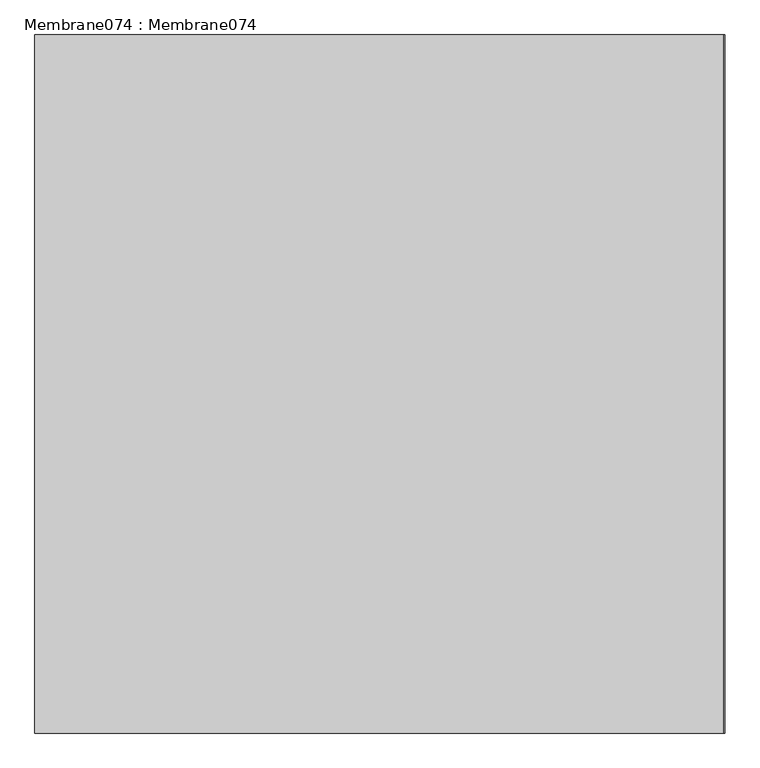
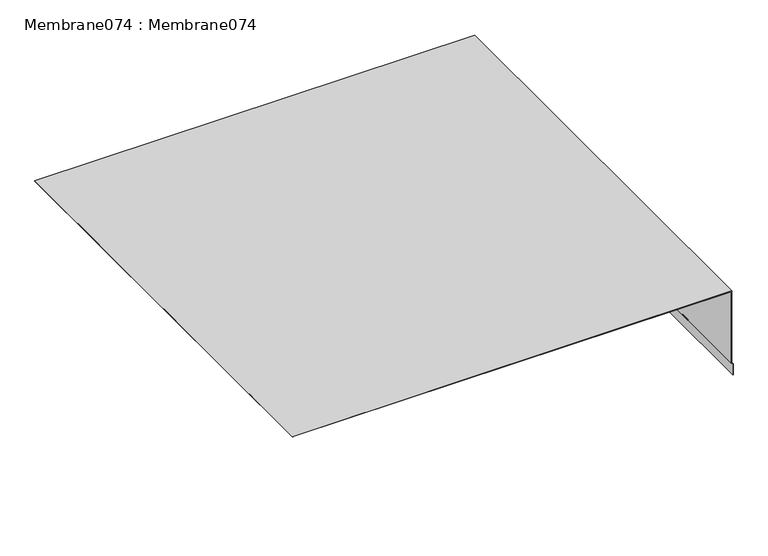
"""IFC4 building model written with IfcOpenShell, lengths in millimetres: proxy geometry, Membrane074 : Membrane074."""

from ifc_helpers import new_model, si_unit, frame, origin, place, context, project, spatial, polyline, outline, extrude, source, transform, mapped, element, save


def membrane074_membrane074_6a089782(model_context):
    return source(origin(), model_context, "Body", "SweptSolid", [
        extrude(outline(polyline([(41765.5156643, 6152.9411918), (41425.552531, 6152.9411918), (41420.2431049, 6158.2506179), (41368.3607574, 6158.2506179), (41368.3607574, 6160.2506179), (41420.9955678, 6160.2506179), (41426.304994, 6154.9411918), (41767.5156643, 6154.9411918), (41767.5156643, 4182.2779227), (41765.5156643, 4182.2779227), (41765.5156643, 6152.9411918)])), frame((0.0, 2217.3609988, 0.0), z_axis=(0.0, 1.0, 0.0), x_axis=(0.0, 0.0, 1.0)), (0.0, 0.0, 1.0), 2000.0),
    ])


if __name__ == "__main__":
    model = new_model("IFC4")
    model_context = context("Model", 3, world=origin())
    ifc_project = project(units=[si_unit("LENGTHUNIT", "METRE", prefix="MILLI")], contexts=[model_context])
    site = spatial("IfcSite", under=ifc_project)
    building = spatial("IfcBuilding", under=site)
    placement = place(None, origin())
    membrane074_membrane074_shape = membrane074_membrane074_6a089782(model_context)
    element("IfcBuildingElementProxy", 1, Name="Membrane074 : Membrane074", ObjectType="Membrane074 : Membrane074", at=placement, inside=building, context=model_context, shape_type="MappedRepresentation", body=[
        mapped(membrane074_membrane074_shape, transform((0.0, 0.0, 0.0), x_axis=(1.0, 0.0, 0.0), y_axis=(0.0, 1.0, 0.0), z_axis=(0.0, 0.0, 1.0))),
    ])
    save(model, "model.ifc")

# Revit data of these elements
# Type "Membrane074 : Membrane074"
#   NameOverride = "Membrane074"
# Element 1 (IfcBuildingElementProxy, "Membrane074 : Membrane074")
#   Materials on its faces: "ASPHALT SATURATED ORGANIC FELT @ ROOF"
# Materials
#   "ASPHALT SATURATED ORGANIC FELT @ ROOF": class "Unassigned", colour RGB 85 170 127, transparency 0
